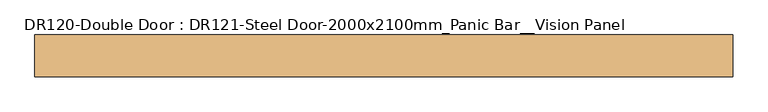
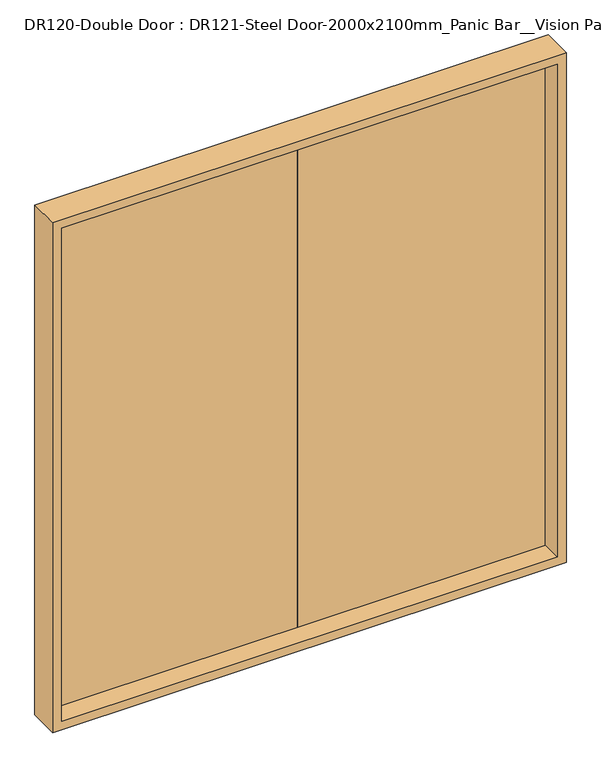
"""IFC4 building model written with IfcOpenShell, lengths in millimetres: door geometry, DR120-Double Door : DR121-Steel Door-2000x2100mm_Panic Bar__Vision Panel."""

from ifc_helpers import new_model, si_unit, frame, origin, place, context, project, spatial, polyline, outline, extrude, faceted_brep, source, transform, mapped, element, save


def dr120_double_door_dr121_steel_door_2000x2100mm_panic_bar_0ab44dcc(model_context):
    return source(origin(), model_context, "Body", "SolidModel", [
        extrude(outline(polyline([(980.0, 20.0), (0.0, 20.0), (0.0, 60.0), (980.0, 60.0), (980.0, 20.0)])), frame((0.0, 0.0, 20.0), z_axis=(0.0, 0.0, 1.0), x_axis=(1.0, 0.0, 0.0)), (0.0, 0.0, 1.0), 2060.0),
        extrude(outline(polyline([(0.0, 20.0), (-980.0, 20.0), (-980.0, 60.0), (0.0, 60.0), (0.0, 20.0)])), frame((0.0, 0.0, 20.0), z_axis=(0.0, 0.0, 1.0), x_axis=(1.0, 0.0, 0.0)), (0.0, 0.0, 1.0), 2060.0),
        faceted_brep([(1000.0, -60.0, 2100.0), (1000.0, 60.0, 2100.0), (-1000.0, 60.0, 2100.0), (-1000.0, -60.0, 2100.0), (965.0, 20.0, 2065.0), (965.0, -60.0, 2065.0), (-965.0, -60.0, 2065.0), (-965.0, 20.0, 2065.0), (980.0, 60.0, 2080.0), (980.0, 20.0, 2080.0), (-980.0, 20.0, 2080.0), (-980.0, 60.0, 2080.0), (-1000.0, 60.0, 0.0), (-1000.0, -60.0, 0.0), (-965.0, -60.0, 35.0), (-965.0, 20.0, 35.0), (-980.0, 20.0, 20.0), (-980.0, 60.0, 20.0), (1000.0, 60.0, 0.0), (980.0, 60.0, 20.0), (1000.0, -60.0, 0.0), (965.0, -60.0, 35.0), (965.0, 20.0, 35.0), (980.0, 20.0, 20.0)], [[[0, 1, 2, 3]], [[4, 5, 6, 7]], [[8, 9, 10, 11]], [[3, 2, 12, 13]], [[7, 6, 14, 15]], [[11, 10, 16, 17]], [[18, 12, 2, 1], [8, 11, 17, 19]], [[13, 12, 18, 20]], [[0, 3, 13, 20], [21, 14, 6, 5]], [[15, 14, 21, 22]], [[23, 16, 10, 9], [4, 7, 15, 22]], [[17, 16, 23, 19]], [[20, 18, 1, 0]], [[22, 21, 5, 4]], [[19, 23, 9, 8]]]),
    ])


if __name__ == "__main__":
    model = new_model("IFC4")
    model_context = context("Model", 3, world=origin())
    ifc_project = project(units=[si_unit("LENGTHUNIT", "METRE", prefix="MILLI")], contexts=[model_context])
    site = spatial("IfcSite", under=ifc_project)
    building = spatial("IfcBuilding", under=site)
    placement = place(None, origin())
    dr120_double_door_dr121_steel_door_2000x2100mm_panic_bar_shape = dr120_double_door_dr121_steel_door_2000x2100mm_panic_bar_0ab44dcc(model_context)
    element("IfcDoor", 1, ObjectType="DR120-Double Door : DR121-Steel Door-2000x2100mm_Panic Bar__Vision Panel", at=placement, inside=building, context=model_context, shape_type="MappedRepresentation", body=[
        mapped(dr120_double_door_dr121_steel_door_2000x2100mm_panic_bar_shape, transform((0.0, 0.0, 0.0), x_axis=(1.0, 0.0, 0.0), y_axis=(0.0, 1.0, 0.0), z_axis=(0.0, 0.0, 1.0))),
    ])
    save(model, "model.ifc")

# Revit data of these elements
# Type "DR120-Double Door : DR121-Steel Door-2000x2100mm_Panic Bar__Vision Panel"
#   Type Mark = "SD"
#   프레임 = ""
#   철물 = ""
#   유리/마감 = ""
#   위치/개소 = ""
#   부호 = "1/SD"
#   문번호 = ""
#   문기호 = "SD"
#   Analytic Construction = "<None>"
#   Height = 2.1000 m
#   Width = 2.0000 m
#   Define Thermal Properties by = 1
#   문 틀 = none
#   문 = none
#   Function = (empty or 0)
#   Assembly Code = ""
#   Wall Closure = (empty or 0)
